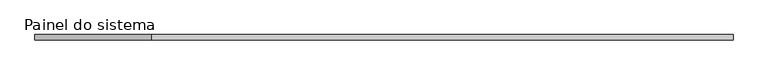
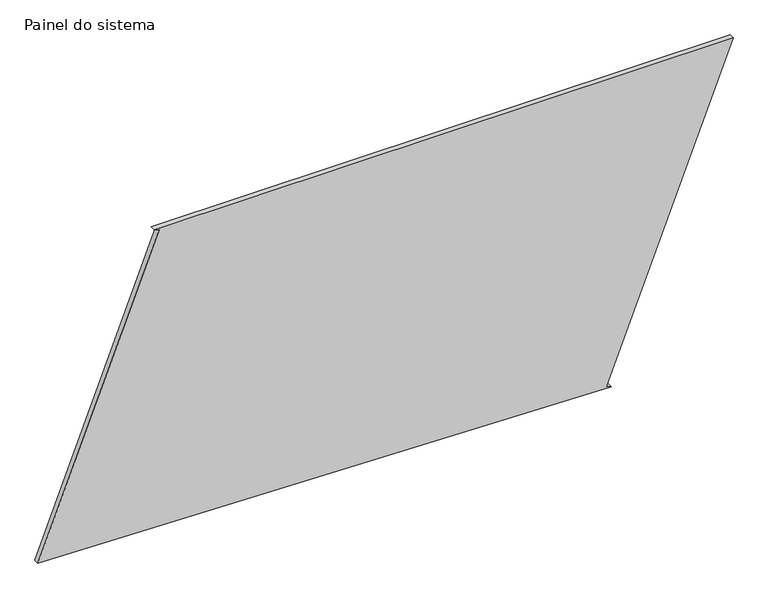
"""IFC4 building model written with IfcOpenShell, lengths in millimetres: plate geometry, Painel do sistema : Envidraçado."""

import ifcopenshell
import ifcopenshell.guid

model = None  # the IFC model being written
_history = None  # IfcOwnerHistory: only IFC2X3 demands one
_inside = {}  # id of a spatial element -> (the spatial element, [elements in it])
_under = {}  # id of a project, library or spatial element -> (it, [spatial elements below it])
_declared = {}  # id of a project -> (the project, [libraries it declares])
_typed = {}  # id of a type object -> (the type object, [elements of that type])
_made_of = {}  # id of a material, layer set ... -> (it, [elements and type objects made of it])


def new_model(schema):
    """Start an empty IFC model of exactly this schema.

    Asked for "IFC4X3", IfcOpenShell would pick the latest addendum, in which some entities
    have other attributes; the version numbers below select the first issue.
    IFC2X3 requires an IfcOwnerHistory on every rooted entity: one is made here for all.
    """
    global model, _history
    if schema == "IFC4X3":
        model = ifcopenshell.file(schema_version=(4, 3, 0, 0))
    else:
        model = ifcopenshell.file(schema=schema)
    _inside.clear()
    _under.clear()
    _declared.clear()
    _typed.clear()
    _made_of.clear()
    _history = None
    if model.schema == "IFC2X3":
        org = make("IfcOrganization", Name="unknown")
        user = make(
            "IfcPersonAndOrganization",
            ThePerson=make("IfcPerson", FamilyName="unknown"),
            TheOrganization=org,
        )
        app = make(
            "IfcApplication",
            ApplicationDeveloper=org,
            Version="unknown",
            ApplicationFullName="unknown",
            ApplicationIdentifier="unknown",
        )
        _history = make(
            "IfcOwnerHistory",
            OwningUser=user,
            OwningApplication=app,
            ChangeAction="ADDED",
            CreationDate=0,
        )
    return model


def make(cls, **values):
    """One entity of the class cls with the attributes given. An attribute that is None is left unset."""
    return model.create_entity(
        cls, **{name: value for name, value in values.items() if value is not None}
    )


def rooted(cls, **values):
    """An entity with a GlobalId (a new one), such as an element, a storey or a relation."""
    return make(cls, GlobalId=ifcopenshell.guid.new(), OwnerHistory=_history, **values)


def si_unit(unit_type, name, prefix=None):
    """IfcSIUnit, for example si_unit("LENGTHUNIT", "METRE", prefix="MILLI")."""
    return make("IfcSIUnit", UnitType=unit_type, Prefix=prefix, Name=name)


def assignment(units):
    """IfcUnitAssignment: the units of a project."""
    return None if units is None else make("IfcUnitAssignment", Units=units)


def point(xyz):
    """IfcCartesianPoint."""
    return None if xyz is None else make("IfcCartesianPoint", Coordinates=xyz)


def direction(xyz):
    """IfcDirection."""
    return None if xyz is None else make("IfcDirection", DirectionRatios=xyz)


def frame(location, z_axis=None, x_axis=None):
    """IfcAxis2Placement3D, a coordinate frame: its origin and axes. An axis left out is left unset."""
    return make(
        "IfcAxis2Placement3D",
        Location=point(location),
        Axis=direction(z_axis),
        RefDirection=direction(x_axis),
    )


def origin():
    """The frame at (0, 0, 0) with its axes left unset."""
    return frame((0.0, 0.0, 0.0))


def place(relative_to, where):
    """IfcLocalPlacement: puts the frame where relative to a parent placement (None: the world)."""
    return make(
        "IfcLocalPlacement", PlacementRelTo=relative_to, RelativePlacement=where
    )


def context(
    kind, dimensions, precision=None, world=None, true_north=None, identifier=None
):
    """IfcGeometricRepresentationContext, for example the 3D "Model" context."""
    return make(
        "IfcGeometricRepresentationContext",
        ContextIdentifier=identifier,
        ContextType=kind,
        CoordinateSpaceDimension=dimensions,
        Precision=precision,
        WorldCoordinateSystem=world,
        TrueNorth=true_north,
    )


def project(units=None, contexts=None):
    """IfcProject with its units and contexts."""
    return rooted(
        "IfcProject",
        Name="project",
        RepresentationContexts=contexts,
        UnitsInContext=assignment(units),
    )


def spatial(cls, under=None, at=None, **own):
    """A site, building, storey or space (cls), placed at a placement, below another one or the project."""
    s = rooted(cls, ObjectPlacement=at, **own)
    if under is not None:
        _under.setdefault(under.id(), (under, []))[1].append(s)
    return s


def polyline(points):
    """IfcPolyline through the points."""
    return make("IfcPolyline", Points=[point(p) for p in points])


def outline(outer, holes=None, kind="AREA"):
    """IfcArbitraryClosedProfileDef: a profile drawn as a closed curve; with holes, ...WithVoids."""
    if holes is None:
        return make("IfcArbitraryClosedProfileDef", ProfileType=kind, OuterCurve=outer)
    return make(
        "IfcArbitraryProfileDefWithVoids",
        ProfileType=kind,
        OuterCurve=outer,
        InnerCurves=holes,
    )


def extrude(swept, where, along, depth):
    """IfcExtrudedAreaSolid: the profile swept, set in the frame where, extruded along a direction by depth."""
    return make(
        "IfcExtrudedAreaSolid",
        SweptArea=swept,
        Position=where,
        ExtrudedDirection=direction(along),
        Depth=depth,
    )


def shape(context_of_items, identifier, shape_type, items):
    """IfcShapeRepresentation: the items that make up one representation, for example the "Body"."""
    return make(
        "IfcShapeRepresentation",
        ContextOfItems=context_of_items,
        RepresentationIdentifier=identifier,
        RepresentationType=shape_type,
        Items=items,
    )


def source(mapping_origin, context_of_items, identifier, shape_type, items):
    """IfcRepresentationMap: a shape defined once, which mapped items show again and again."""
    return make(
        "IfcRepresentationMap",
        MappingOrigin=mapping_origin,
        MappedRepresentation=shape(context_of_items, identifier, shape_type, items),
    )


def transform(
    local_origin,
    x_axis=None,
    y_axis=None,
    z_axis=None,
    scale=None,
    scale2=None,
    scale3=None,
    uniform=True,
):
    """IfcCartesianTransformationOperator3D, or its non-uniform kind. x_axis, y_axis, z_axis: its Axis1, 2, 3."""
    if uniform:
        return make(
            "IfcCartesianTransformationOperator3D",
            Axis1=direction(x_axis),
            Axis2=direction(y_axis),
            LocalOrigin=point(local_origin),
            Scale=scale,
            Axis3=direction(z_axis),
        )
    return make(
        "IfcCartesianTransformationOperator3DnonUniform",
        Axis1=direction(x_axis),
        Axis2=direction(y_axis),
        LocalOrigin=point(local_origin),
        Scale=scale,
        Axis3=direction(z_axis),
        Scale2=scale2,
        Scale3=scale3,
    )


def mapped(mapping_source, mapping_target):
    """IfcMappedItem: shows the shape of a source again, moved by a transform."""
    return make(
        "IfcMappedItem", MappingSource=mapping_source, MappingTarget=mapping_target
    )


def made_of(thing, what):
    """Note that an element or type object is made of a material, layer set ...; save() writes the relation."""
    if what is not None:
        _made_of.setdefault(what.id(), (what, []))[1].append(thing)
    return thing


def element(
    cls,
    number,
    at=None,
    inside=None,
    cuts=None,
    type_object=None,
    material=None,
    context=None,
    identifier="Body",
    shape_type=None,
    held_by="IfcProductDefinitionShape",
    body=None,
    shapes=None,
    **own,
):
    """One element of the class cls, such as IfcWall. Its Tag is "e" and its number.

    at: its placement. inside: the storey or other place that contains it. cuts: it is an
    opening in that element (IfcRelVoidsElement). A single representation is given by context,
    identifier, shape_type and body (its items); several are given by shapes. held_by: the class
    of the entity that holds the representations. save() writes the other relations.
    """
    e = rooted(cls, Tag="e%d" % number, ObjectPlacement=at, **own)
    if body is not None:
        shapes = [shape(context, identifier, shape_type, body)]
    if shapes is not None:
        e.Representation = make(held_by, Representations=shapes)
    if inside is not None:
        _inside.setdefault(inside.id(), (inside, []))[1].append(e)
    if cuts is not None:
        rooted(
            "IfcRelVoidsElement", RelatingBuildingElement=cuts, RelatedOpeningElement=e
        )
    if type_object is not None:
        _typed.setdefault(type_object.id(), (type_object, []))[1].append(e)
    return made_of(e, material)


def aggregate(whole, parts):
    """IfcRelAggregates: a whole, such as a stair, and the parts it consists of."""
    return rooted("IfcRelAggregates", RelatingObject=whole, RelatedObjects=parts)


def save(model, path):
    """Write the relations noted so far, then the file.

    IfcRelAggregates (storeys below a building ...), IfcRelContainedInSpatialStructure (elements
    in a storey), IfcRelDefinesByType, IfcRelAssociatesMaterial and IfcRelDeclares: one each for
    every whole, place, type object, material and project.
    """
    for whole, parts in _under.values():
        aggregate(whole, parts)
    for where, things in _inside.values():
        rooted(
            "IfcRelContainedInSpatialStructure",
            RelatedElements=things,
            RelatingStructure=where,
        )
    for kind, things in _typed.values():
        rooted("IfcRelDefinesByType", RelatedObjects=things, RelatingType=kind)
    for what, things in _made_of.values():
        rooted("IfcRelAssociatesMaterial", RelatedObjects=things, RelatingMaterial=what)
    for by, libraries in _declared.values():
        rooted("IfcRelDeclares", RelatingContext=by, RelatedDefinitions=libraries)
    model.write(path)


def painel_do_sistema_520132bf(model_context):
    return source(origin(), model_context, "Body", "SweptSolid", [
        extrude(outline(polyline([(0.0, 1066.4854985), (9.0972802, 1043.1994621), (1541.5058722, 1641.8737131), (1541.5058722, -1093.2728918), (1532.4085919, -1069.9868553), (68.5668902, -1641.8737131), (0.0, 1066.4854985)])), frame((0.0, 24.5, 0.0), z_axis=(0.0, 1.0, 0.0), x_axis=(0.0, 0.0, 1.0)), (0.0, 0.0, 1.0), 25.0),
    ])


if __name__ == "__main__":
    model = new_model("IFC4")
    model_context = context("Model", 3, world=origin())
    ifc_project = project(units=[si_unit("LENGTHUNIT", "METRE", prefix="MILLI")], contexts=[model_context])
    site = spatial("IfcSite", under=ifc_project)
    building = spatial("IfcBuilding", under=site)
    placement = place(None, origin())
    painel_do_sistema_shape = painel_do_sistema_520132bf(model_context)
    element("IfcPlate", 1, ObjectType="Painel do sistema : Envidraçado", at=placement, inside=building, context=model_context, shape_type="MappedRepresentation", body=[
        mapped(painel_do_sistema_shape, transform((0.0, 0.0, 0.0), x_axis=(1.0, 0.0, 0.0), y_axis=(0.0, 1.0, 0.0), z_axis=(0.0, 0.0, 1.0))),
    ])
    save(model, "model.ifc")

# Revit data of these elements
# Type "Painel do sistema : Envidraçado"
#   Construction Type Id = "GSP4R"
#   Analytic Construction = "Vidraça única Pilkington 1/8 pol"
#   Visual Light Transmittance = 0.9
#   Solar Heat Gain Coefficient = 0.86
#   Heat Transfer Coefficient (U) = 6.7069 W/(m²·K)
# Element 1 (IfcPlate, "Painel do sistema : Envidraçado")
#   Materials on its faces: "Vidro"
# Materials
#   "Vidro": class "Vidro", colour RGB 0 128 192, transparency 0.9, Description = "Vidro de sílica", Cost = 0
